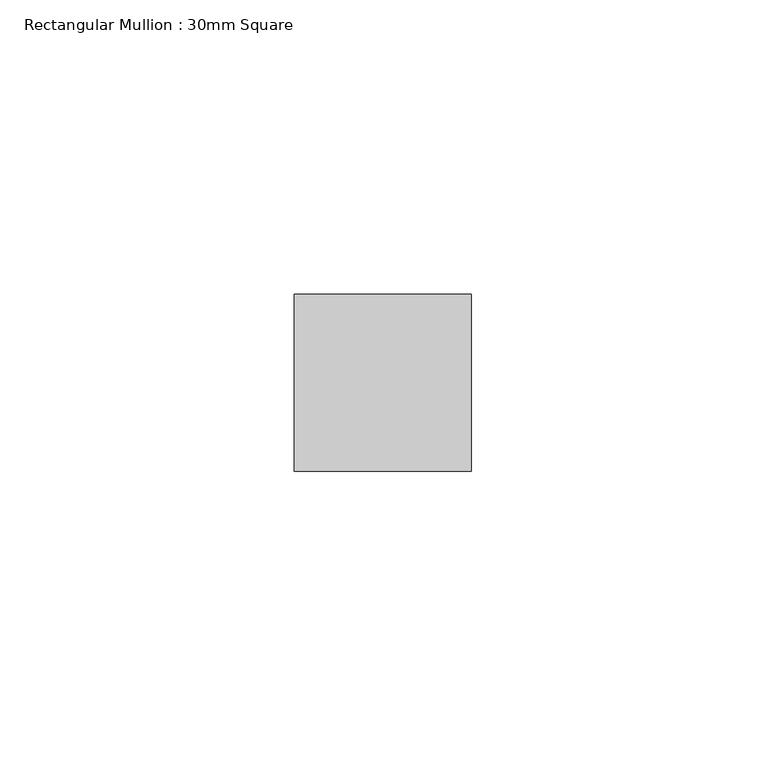
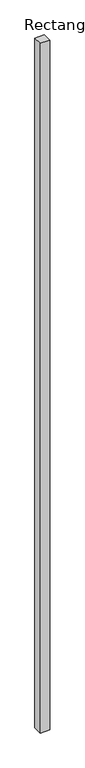
"""IFC4 building model written with IfcOpenShell, lengths in millimetres: member geometry, Rectangular Mullion : 30mm Square."""

from ifc_helpers import new_model, si_unit, frame, origin, place, context, project, spatial, polyline, outline, extrude, source, transform, mapped, element, save


def rectangular_mullion_30mm_square_25ecd6b2(model_context):
    return source(origin(), model_context, "Body", "SweptSolid", [
        extrude(outline(polyline([(15.0, 15.0), (15.0, -15.0), (-15.0, -15.0), (-15.0, 15.0), (15.0, 15.0)])), frame((0.0, 0.0, -2311.5857878), z_axis=(0.0, 0.0, 1.0), x_axis=(1.0, 0.0, 0.0)), (0.0, 0.0, 1.0), 2311.5857878),
    ])


if __name__ == "__main__":
    model = new_model("IFC4")
    model_context = context("Model", 3, world=origin())
    ifc_project = project(units=[si_unit("LENGTHUNIT", "METRE", prefix="MILLI")], contexts=[model_context])
    site = spatial("IfcSite", under=ifc_project)
    building = spatial("IfcBuilding", under=site)
    placement = place(None, origin())
    rectangular_mullion_30mm_square_shape = rectangular_mullion_30mm_square_25ecd6b2(model_context)
    element("IfcMember", 1, ObjectType="Rectangular Mullion : 30mm Square", at=placement, inside=building, context=model_context, shape_type="MappedRepresentation", body=[
        mapped(rectangular_mullion_30mm_square_shape, transform((0.0, 0.0, 0.0), x_axis=(1.0, 0.0, 0.0), y_axis=(0.0, 1.0, 0.0), z_axis=(0.0, 0.0, 1.0))),
    ])
    save(model, "model.ifc")

# Revit data of these elements
# Type "Rectangular Mullion : 30mm Square"
#   built-in parameter 1007304 = 0.0984252 (stored number, unit not read)
#   built-in parameter 1007301 = 0.0492126 (stored number, unit not read)
#   built-in parameter 1007300 = 0.0492126 (stored number, unit not read)
# Element 1 (IfcMember, "Rectangular Mullion : 30mm Square")
#   Materials on its faces: "Aluminum"
# Materials
#   "Aluminum": class "Metal", colour RGB 244 244 244, transparency 0, Description = "Aluminum 6061", Cost = 0
